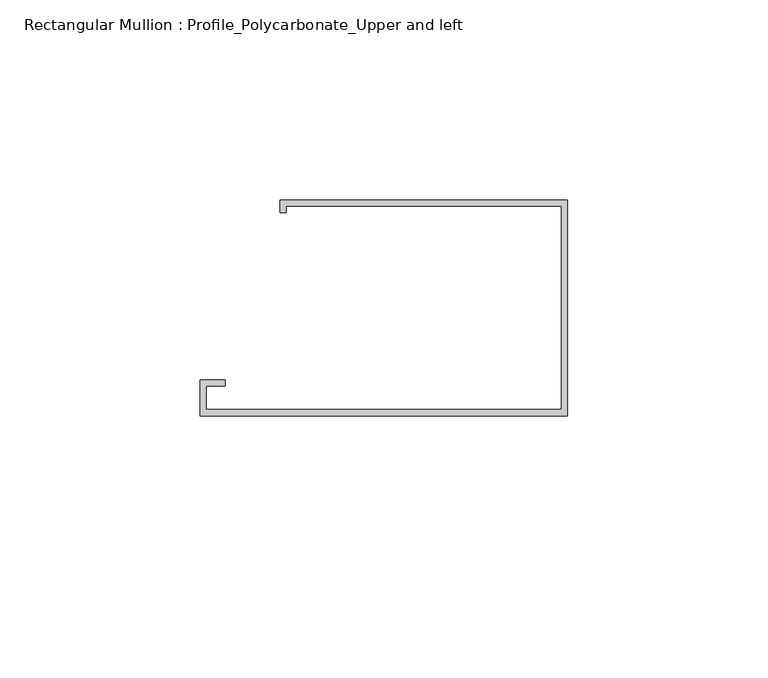
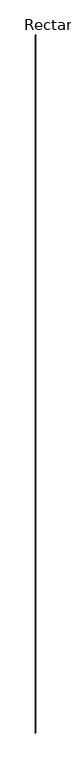
"""IFC4 building model written with IfcOpenShell, lengths in millimetres: member geometry, Rectangular Mullion : Profile_Polycarbonate_Upper and left."""

from ifc_helpers import new_model, si_unit, frame, origin, place, context, project, spatial, polyline, outline, extrude, source, transform, mapped, element, save


def rectangular_mullion_profile_polycarbonate_upper_and_left_b00cdadc(model_context):
    return source(origin(), model_context, "Body", "SweptSolid", [
        extrude(outline(polyline([(0.0, -28.984575), (-91.9988, -28.984575), (-91.9988, -19.992975), (-85.6488, -19.992975), (-85.6488, -21.580475), (-90.4113, -21.580475), (-90.4113, -27.397075), (-1.5875, -27.397075), (-1.5875, 23.428325), (-70.3961, 23.428325), (-70.3961, 21.840825), (-71.9836, 21.840825), (-71.9836, 25.015825), (0.0, 25.015825), (0.0, -28.984575)])), frame((0.0, 0.0, -88808.486975), z_axis=(0.0, 0.0, 1.0), x_axis=(1.0, 0.0, 0.0)), (0.0, 0.0, 1.0), 88808.486975),
    ])


if __name__ == "__main__":
    model = new_model("IFC4")
    model_context = context("Model", 3, world=origin())
    ifc_project = project(units=[si_unit("LENGTHUNIT", "METRE", prefix="MILLI")], contexts=[model_context])
    site = spatial("IfcSite", under=ifc_project)
    building = spatial("IfcBuilding", under=site)
    placement = place(None, origin())
    rectangular_mullion_profile_polycarbonate_upper_and_left_shape = rectangular_mullion_profile_polycarbonate_upper_and_left_b00cdadc(model_context)
    element("IfcMember", 1, ObjectType="Rectangular Mullion : Profile_Polycarbonate_Upper and left", at=placement, inside=building, context=model_context, shape_type="MappedRepresentation", body=[
        mapped(rectangular_mullion_profile_polycarbonate_upper_and_left_shape, transform((0.0, 0.0, 0.0), x_axis=(1.0, 0.0, 0.0), y_axis=(0.0, 1.0, 0.0), z_axis=(0.0, 0.0, 1.0))),
    ])
    save(model, "model.ifc")

# Revit data of these elements
# Type "Rectangular Mullion : Profile_Polycarbonate_Upper and left"
#   built-in parameter 1007322 = 0.177167 (stored number, unit not read)
#   built-in parameter 1007321 = 0.00520833 (stored number, unit not read)
#   built-in parameter 1007320 = 0 (stored number, unit not read)
